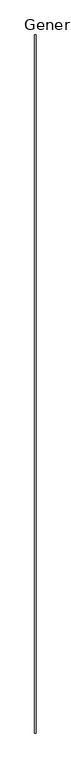
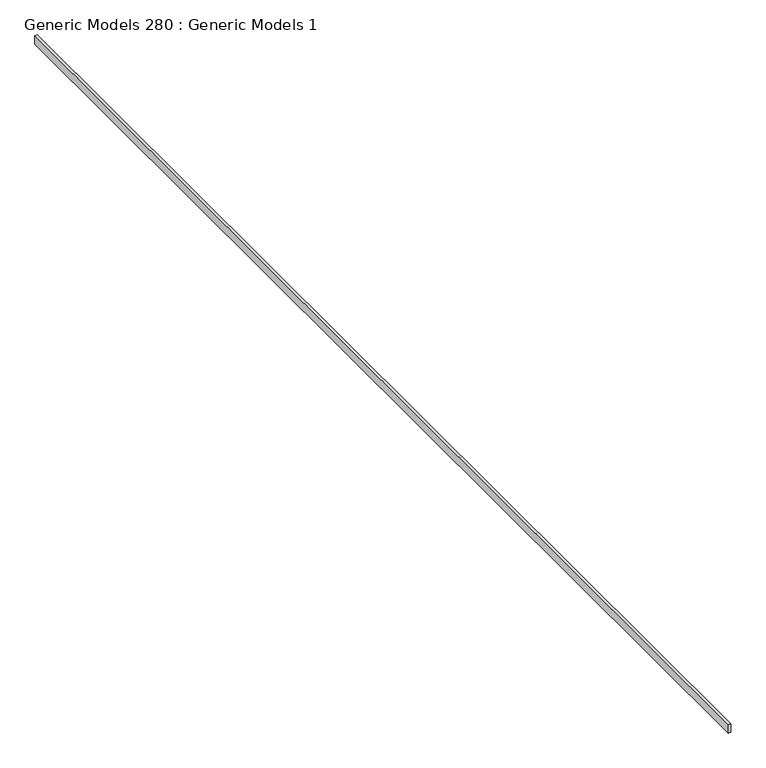
"""IFC4 building model written with IfcOpenShell, lengths in millimetres: proxy geometry, Generic Models 280 : Generic Models 1."""

from ifc_helpers import new_model, si_unit, frame, origin, place, context, project, spatial, polyline, outline, extrude, source, transform, mapped, element, save


def generic_models_280_generic_models_1_3dc5fd40(model_context):
    return source(origin(), model_context, "Body", "SweptSolid", [
        extrude(outline(polyline([(4762.3263704, 16178.0560596), (4800.4263704, 16178.0560596), (4800.4263704, -2871.9439404), (4762.3263704, -2871.9439404), (4762.3263704, 16178.0560596)])), frame((0.0, 0.0, 124770.896), z_axis=(0.0, 0.0, 1.0), x_axis=(1.0, 0.0, 0.0)), (0.0, 0.0, 1.0), 139.7),
    ])


if __name__ == "__main__":
    model = new_model("IFC4")
    model_context = context("Model", 3, world=origin())
    ifc_project = project(units=[si_unit("LENGTHUNIT", "METRE", prefix="MILLI")], contexts=[model_context])
    site = spatial("IfcSite", under=ifc_project)
    building = spatial("IfcBuilding", under=site)
    placement = place(None, origin())
    generic_models_280_generic_models_1_shape = generic_models_280_generic_models_1_3dc5fd40(model_context)
    element("IfcBuildingElementProxy", 1, Name="Generic Models 280 : Generic Models 1", ObjectType="Generic Models 280 : Generic Models 1", at=placement, inside=building, context=model_context, shape_type="MappedRepresentation", body=[
        mapped(generic_models_280_generic_models_1_shape, transform((0.0, 0.0, 0.0), x_axis=(1.0, 0.0, 0.0), y_axis=(0.0, 1.0, 0.0), z_axis=(0.0, 0.0, 1.0))),
    ])
    save(model, "model.ifc")

# Revit data of these elements
# Element 1 (IfcBuildingElementProxy, "Generic Models 280 : Generic Models 1")
#   Materials on its faces: "_2X BLOCKING AS REQUIRED"
# Materials
#   "_2X BLOCKING AS REQUIRED": class "Generic", colour RGB 177 130 114, transparency 0, Cost = 0
